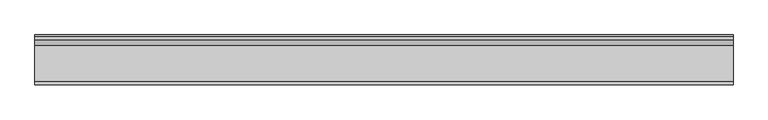
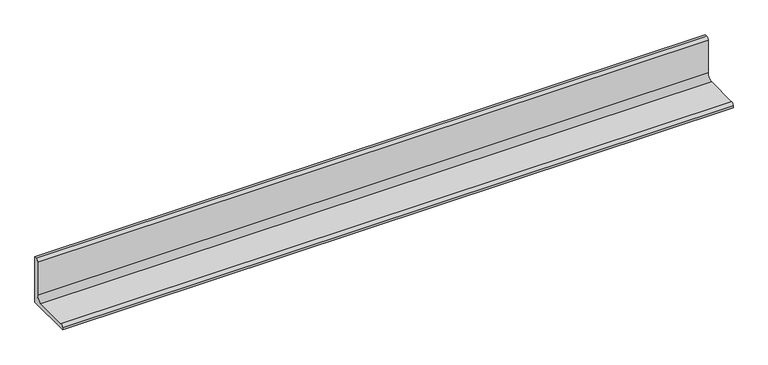
"""IFC4 building model written with IfcOpenShell, lengths in millimetres: beam geometry, NLRS_28_SF_LIB_stalen ligger hoekprofiel gelijkzijdig-AV-MMBS-SRP_gen_rsf : stalen ligger gelijkzijdig hoekprofiel LEQU_gen__100x100x10."""

from ifc_helpers import new_model, si_unit, point, frame, frame_2d, origin, place, context, project, spatial, polyline, circle_curve, trimmed, segment, composite_curve, outline, extrude, source, transform, mapped, element, save


def beam_757c45da(model_context):
    return source(origin(), model_context, "Body", "SweptSolid", [
        extrude(outline(composite_curve([segment(polyline([(28.22, -28.22), (-71.78, -28.22), (-71.78, -24.22)]), True, "CONTINUOUS"), segment(trimmed(circle_curve(frame_2d((-65.78, -24.22)), 6.0), [point((-71.78, -24.22))], [point((-65.78, -18.22))], False, "CARTESIAN"), True, "CONTINUOUS"), segment(polyline([(-65.78, -18.22), (6.22, -18.22)]), True, "CONTINUOUS"), segment(trimmed(circle_curve(frame_2d((6.22, -6.22)), 12.0), [point((6.22, -18.22))], [point((18.22, -6.22))], True, "CARTESIAN"), True, "CONTINUOUS"), segment(polyline([(18.22, -6.22), (18.22, 65.78)]), True, "CONTINUOUS"), segment(trimmed(circle_curve(frame_2d((24.22, 65.78)), 6.0), [point((18.22, 65.78))], [point((24.22, 71.78))], False, "CARTESIAN"), True, "CONTINUOUS"), segment(polyline([(24.22, 71.78), (28.22, 71.78), (28.22, -28.22)]), True, "CONTINUOUS")], self_intersect=False)), frame((-700.0, 0.0, 0.0), z_axis=(1.0, 0.0, 0.0), x_axis=(0.0, 1.0, 0.0)), (0.0, 0.0, 1.0), 1400.0),
    ])


if __name__ == "__main__":
    model = new_model("IFC4")
    model_context = context("Model", 3, world=origin())
    ifc_project = project(units=[si_unit("LENGTHUNIT", "METRE", prefix="MILLI")], contexts=[model_context])
    site = spatial("IfcSite", under=ifc_project)
    building = spatial("IfcBuilding", under=site)
    placement = place(None, origin())
    beam_shape = beam_757c45da(model_context)
    element("IfcBeam", 1, ObjectType="NLRS_28_SF_LIB_stalen ligger hoekprofiel gelijkzijdig-AV-MMBS-SRP_gen_rsf : stalen ligger gelijkzijdig hoekprofiel LEQU_gen__100x100x10", at=placement, inside=building, context=model_context, shape_type="MappedRepresentation", body=[
        mapped(beam_shape, transform((0.0, 0.0, 0.0), x_axis=(1.0, 0.0, 0.0), y_axis=(0.0, 1.0, 0.0), z_axis=(0.0, 0.0, 1.0))),
    ])
    save(model, "model.ifc")

# Revit data of these elements
# Type "NLRS_28_SF_LIB_stalen ligger hoekprofiel gelijkzijdig-AV-MMBS-SRP_gen_rsf : stalen ligger gelijkzijdig hoekprofiel LEQU_gen__100x100x10"
#   Type IfcGUID = "2CEqVLPNH8KRN7ghwV3a0q"
#   IfcExportAs = "IfcBeamType"
#   Type Comments = "L100x100x10"
#   Model = " "
#   Manufacturer = " "
#   Fire Rating = " "
#   Description = "stalen ligger L100x100x10"
#   Assembly Code = "28.11"
#   vz = 71.78 mm
#   vy = 71.78 mm
#   tw = 10 mm
#   tf = 10 mm
#   ri = 6 mm
#   ra = 12 mm
#   d = 100 mm
#   bf = 100 mm
#   NLRS_C_lengte [instance default] = 1524 mm
#   Length [instance default] = 1524 mm
#   Structural Material = NLRS_h2_staal_gen_rsf
#   Keynote = ""
# Element 1 (IfcBeam, "NLRS_28_SF_LIB_stalen ligger hoekprofiel gelijkzijdig-AV-MMBS-SRP_gen_rsf : stalen ligger gelijkzijdig hoekprofiel LEQU_gen__100x100x10")
#   NLRS_C_lengte = 1400 mm
#   Materials on its faces: "NLRS_h2_staal_gen_rsf"
# Materials
#   "NLRS_h2_staal_gen_rsf": class "H - Metaal", colour RGB 189 187 185, transparency 0, Keynote = "h2", Manufacturer = "Revit Standards Foundation", URL = "www.revitstandards.org", Description = "staal", Cost = 0
